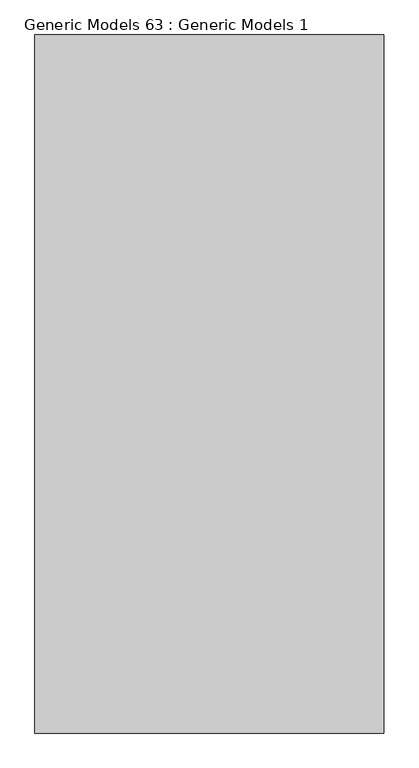
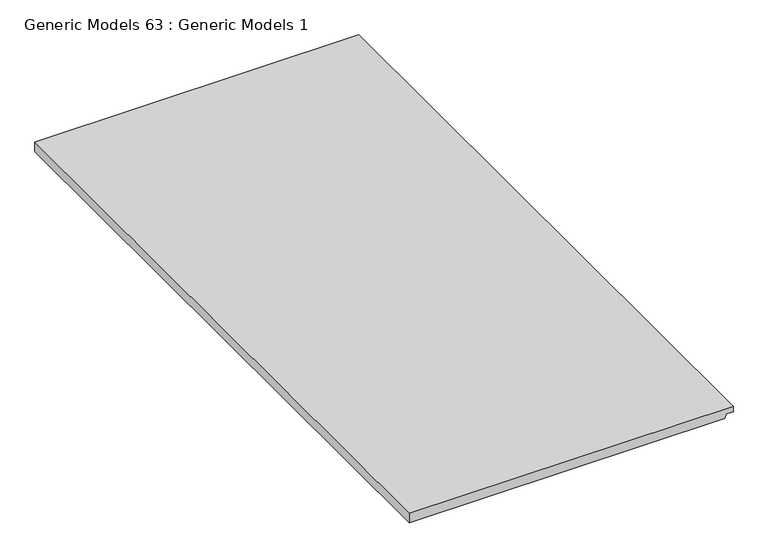
"""IFC4 building model written with IfcOpenShell, lengths in millimetres: proxy geometry, Generic Models 63 : Generic Models 1."""

import ifcopenshell
import ifcopenshell.guid

model = None  # the IFC model being written
_history = None  # IfcOwnerHistory: only IFC2X3 demands one
_inside = {}  # id of a spatial element -> (the spatial element, [elements in it])
_under = {}  # id of a project, library or spatial element -> (it, [spatial elements below it])
_declared = {}  # id of a project -> (the project, [libraries it declares])
_typed = {}  # id of a type object -> (the type object, [elements of that type])
_made_of = {}  # id of a material, layer set ... -> (it, [elements and type objects made of it])


def new_model(schema):
    """Start an empty IFC model of exactly this schema.

    Asked for "IFC4X3", IfcOpenShell would pick the latest addendum, in which some entities
    have other attributes; the version numbers below select the first issue.
    IFC2X3 requires an IfcOwnerHistory on every rooted entity: one is made here for all.
    """
    global model, _history
    if schema == "IFC4X3":
        model = ifcopenshell.file(schema_version=(4, 3, 0, 0))
    else:
        model = ifcopenshell.file(schema=schema)
    _inside.clear()
    _under.clear()
    _declared.clear()
    _typed.clear()
    _made_of.clear()
    _history = None
    if model.schema == "IFC2X3":
        org = make("IfcOrganization", Name="unknown")
        user = make(
            "IfcPersonAndOrganization",
            ThePerson=make("IfcPerson", FamilyName="unknown"),
            TheOrganization=org,
        )
        app = make(
            "IfcApplication",
            ApplicationDeveloper=org,
            Version="unknown",
            ApplicationFullName="unknown",
            ApplicationIdentifier="unknown",
        )
        _history = make(
            "IfcOwnerHistory",
            OwningUser=user,
            OwningApplication=app,
            ChangeAction="ADDED",
            CreationDate=0,
        )
    return model


def make(cls, **values):
    """One entity of the class cls with the attributes given. An attribute that is None is left unset."""
    return model.create_entity(
        cls, **{name: value for name, value in values.items() if value is not None}
    )


def rooted(cls, **values):
    """An entity with a GlobalId (a new one), such as an element, a storey or a relation."""
    return make(cls, GlobalId=ifcopenshell.guid.new(), OwnerHistory=_history, **values)


def si_unit(unit_type, name, prefix=None):
    """IfcSIUnit, for example si_unit("LENGTHUNIT", "METRE", prefix="MILLI")."""
    return make("IfcSIUnit", UnitType=unit_type, Prefix=prefix, Name=name)


def assignment(units):
    """IfcUnitAssignment: the units of a project."""
    return None if units is None else make("IfcUnitAssignment", Units=units)


def point(xyz):
    """IfcCartesianPoint."""
    return None if xyz is None else make("IfcCartesianPoint", Coordinates=xyz)


def direction(xyz):
    """IfcDirection."""
    return None if xyz is None else make("IfcDirection", DirectionRatios=xyz)


def frame(location, z_axis=None, x_axis=None):
    """IfcAxis2Placement3D, a coordinate frame: its origin and axes. An axis left out is left unset."""
    return make(
        "IfcAxis2Placement3D",
        Location=point(location),
        Axis=direction(z_axis),
        RefDirection=direction(x_axis),
    )


def origin():
    """The frame at (0, 0, 0) with its axes left unset."""
    return frame((0.0, 0.0, 0.0))


def place(relative_to, where):
    """IfcLocalPlacement: puts the frame where relative to a parent placement (None: the world)."""
    return make(
        "IfcLocalPlacement", PlacementRelTo=relative_to, RelativePlacement=where
    )


def context(
    kind, dimensions, precision=None, world=None, true_north=None, identifier=None
):
    """IfcGeometricRepresentationContext, for example the 3D "Model" context."""
    return make(
        "IfcGeometricRepresentationContext",
        ContextIdentifier=identifier,
        ContextType=kind,
        CoordinateSpaceDimension=dimensions,
        Precision=precision,
        WorldCoordinateSystem=world,
        TrueNorth=true_north,
    )


def project(units=None, contexts=None):
    """IfcProject with its units and contexts."""
    return rooted(
        "IfcProject",
        Name="project",
        RepresentationContexts=contexts,
        UnitsInContext=assignment(units),
    )


def spatial(cls, under=None, at=None, **own):
    """A site, building, storey or space (cls), placed at a placement, below another one or the project."""
    s = rooted(cls, ObjectPlacement=at, **own)
    if under is not None:
        _under.setdefault(under.id(), (under, []))[1].append(s)
    return s


def polyline(points):
    """IfcPolyline through the points."""
    return make("IfcPolyline", Points=[point(p) for p in points])


def outline(outer, holes=None, kind="AREA"):
    """IfcArbitraryClosedProfileDef: a profile drawn as a closed curve; with holes, ...WithVoids."""
    if holes is None:
        return make("IfcArbitraryClosedProfileDef", ProfileType=kind, OuterCurve=outer)
    return make(
        "IfcArbitraryProfileDefWithVoids",
        ProfileType=kind,
        OuterCurve=outer,
        InnerCurves=holes,
    )


def extrude(swept, where, along, depth):
    """IfcExtrudedAreaSolid: the profile swept, set in the frame where, extruded along a direction by depth."""
    return make(
        "IfcExtrudedAreaSolid",
        SweptArea=swept,
        Position=where,
        ExtrudedDirection=direction(along),
        Depth=depth,
    )


def shape(context_of_items, identifier, shape_type, items):
    """IfcShapeRepresentation: the items that make up one representation, for example the "Body"."""
    return make(
        "IfcShapeRepresentation",
        ContextOfItems=context_of_items,
        RepresentationIdentifier=identifier,
        RepresentationType=shape_type,
        Items=items,
    )


def source(mapping_origin, context_of_items, identifier, shape_type, items):
    """IfcRepresentationMap: a shape defined once, which mapped items show again and again."""
    return make(
        "IfcRepresentationMap",
        MappingOrigin=mapping_origin,
        MappedRepresentation=shape(context_of_items, identifier, shape_type, items),
    )


def transform(
    local_origin,
    x_axis=None,
    y_axis=None,
    z_axis=None,
    scale=None,
    scale2=None,
    scale3=None,
    uniform=True,
):
    """IfcCartesianTransformationOperator3D, or its non-uniform kind. x_axis, y_axis, z_axis: its Axis1, 2, 3."""
    if uniform:
        return make(
            "IfcCartesianTransformationOperator3D",
            Axis1=direction(x_axis),
            Axis2=direction(y_axis),
            LocalOrigin=point(local_origin),
            Scale=scale,
            Axis3=direction(z_axis),
        )
    return make(
        "IfcCartesianTransformationOperator3DnonUniform",
        Axis1=direction(x_axis),
        Axis2=direction(y_axis),
        LocalOrigin=point(local_origin),
        Scale=scale,
        Axis3=direction(z_axis),
        Scale2=scale2,
        Scale3=scale3,
    )


def mapped(mapping_source, mapping_target):
    """IfcMappedItem: shows the shape of a source again, moved by a transform."""
    return make(
        "IfcMappedItem", MappingSource=mapping_source, MappingTarget=mapping_target
    )


def made_of(thing, what):
    """Note that an element or type object is made of a material, layer set ...; save() writes the relation."""
    if what is not None:
        _made_of.setdefault(what.id(), (what, []))[1].append(thing)
    return thing


def element(
    cls,
    number,
    at=None,
    inside=None,
    cuts=None,
    type_object=None,
    material=None,
    context=None,
    identifier="Body",
    shape_type=None,
    held_by="IfcProductDefinitionShape",
    body=None,
    shapes=None,
    **own,
):
    """One element of the class cls, such as IfcWall. Its Tag is "e" and its number.

    at: its placement. inside: the storey or other place that contains it. cuts: it is an
    opening in that element (IfcRelVoidsElement). A single representation is given by context,
    identifier, shape_type and body (its items); several are given by shapes. held_by: the class
    of the entity that holds the representations. save() writes the other relations.
    """
    e = rooted(cls, Tag="e%d" % number, ObjectPlacement=at, **own)
    if body is not None:
        shapes = [shape(context, identifier, shape_type, body)]
    if shapes is not None:
        e.Representation = make(held_by, Representations=shapes)
    if inside is not None:
        _inside.setdefault(inside.id(), (inside, []))[1].append(e)
    if cuts is not None:
        rooted(
            "IfcRelVoidsElement", RelatingBuildingElement=cuts, RelatedOpeningElement=e
        )
    if type_object is not None:
        _typed.setdefault(type_object.id(), (type_object, []))[1].append(e)
    return made_of(e, material)


def aggregate(whole, parts):
    """IfcRelAggregates: a whole, such as a stair, and the parts it consists of."""
    return rooted("IfcRelAggregates", RelatingObject=whole, RelatedObjects=parts)


def save(model, path):
    """Write the relations noted so far, then the file.

    IfcRelAggregates (storeys below a building ...), IfcRelContainedInSpatialStructure (elements
    in a storey), IfcRelDefinesByType, IfcRelAssociatesMaterial and IfcRelDeclares: one each for
    every whole, place, type object, material and project.
    """
    for whole, parts in _under.values():
        aggregate(whole, parts)
    for where, things in _inside.values():
        rooted(
            "IfcRelContainedInSpatialStructure",
            RelatedElements=things,
            RelatingStructure=where,
        )
    for kind, things in _typed.values():
        rooted("IfcRelDefinesByType", RelatedObjects=things, RelatingType=kind)
    for what, things in _made_of.values():
        rooted("IfcRelAssociatesMaterial", RelatedObjects=things, RelatingMaterial=what)
    for by, libraries in _declared.values():
        rooted("IfcRelDeclares", RelatingContext=by, RelatedDefinitions=libraries)
    model.write(path)


def generic_models_63_generic_models_1_24b688b4(model_context):
    return source(origin(), model_context, "Body", "SweptSolid", [
        extrude(outline(polyline([(2253.330428, 51977.6676133), (2253.330428, 51368.0676133), (2234.280428, 51368.0676133), (2234.280428, 51962.0785996), (2242.217928, 51964.9676133), (2242.217928, 51977.6676133), (2253.330428, 51977.6676133)])), frame((0.0, 0.0, 0.0), z_axis=(0.0, 1.0, 0.0), x_axis=(0.0, 0.0, 1.0)), (0.0, 0.0, 1.0), 1219.2),
    ])


if __name__ == "__main__":
    model = new_model("IFC4")
    model_context = context("Model", 3, world=origin())
    ifc_project = project(units=[si_unit("LENGTHUNIT", "METRE", prefix="MILLI")], contexts=[model_context])
    site = spatial("IfcSite", under=ifc_project)
    building = spatial("IfcBuilding", under=site)
    placement = place(None, origin())
    generic_models_63_generic_models_1_shape = generic_models_63_generic_models_1_24b688b4(model_context)
    element("IfcBuildingElementProxy", 1, Name="Generic Models 63 : Generic Models 1", ObjectType="Generic Models 63 : Generic Models 1", at=placement, inside=building, context=model_context, shape_type="MappedRepresentation", body=[
        mapped(generic_models_63_generic_models_1_shape, transform((0.0, 0.0, 0.0), x_axis=(1.0, 0.0, 0.0), y_axis=(0.0, 1.0, 0.0), z_axis=(0.0, 0.0, 1.0))),
    ])
    save(model, "model.ifc")

# Revit data of these elements
# Element 1 (IfcBuildingElementProxy, "Generic Models 63 : Generic Models 1")
#   Materials on its faces: "CEILING AS SCHEDULED"
# Materials
#   "CEILING AS SCHEDULED": class "Generic", colour RGB 255 255 255, transparency 0, Cost = 0
